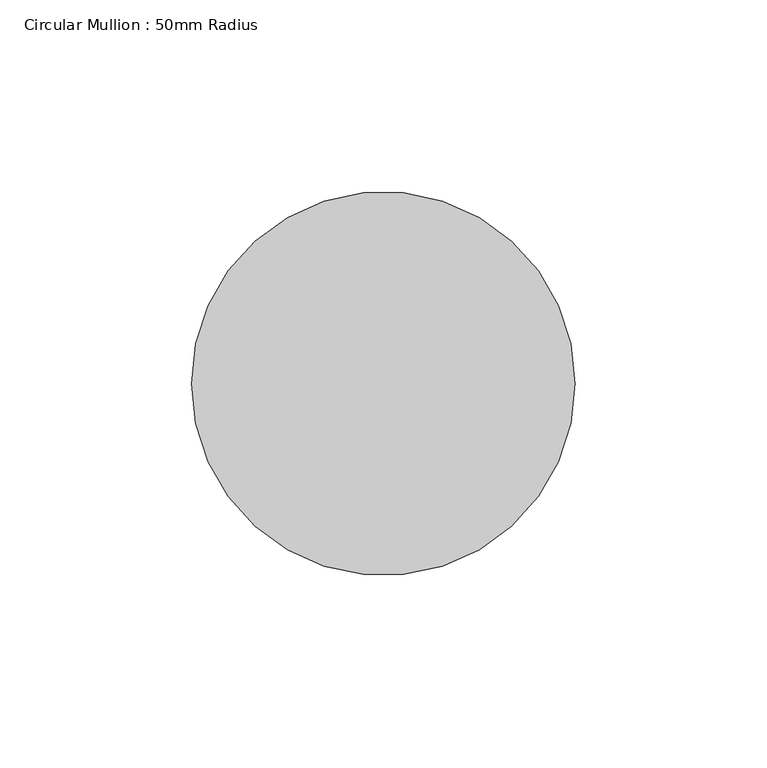
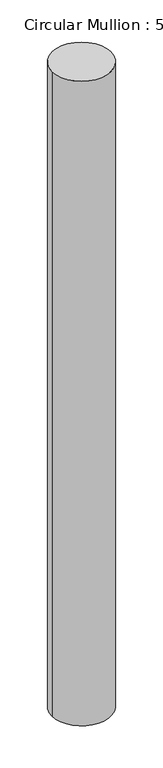
"""IFC4 building model written with IfcOpenShell, lengths in millimetres: member geometry, Circular Mullion : 50mm Radius."""

from ifc_helpers import new_model, si_unit, point, frame, origin, origin_2d, place, context, project, spatial, circle_curve, trimmed, segment, composite_curve, outline, extrude, source, transform, mapped, element, save


def circular_mullion_50mm_radius_acc5950d(model_context):
    return source(origin(), model_context, "Body", "SweptSolid", [
        extrude(outline(composite_curve([segment(trimmed(circle_curve(origin_2d(), 50.0), [point((50.0, 0.0))], [point((-50.0, 0.0))], False, "CARTESIAN"), True, "CONTINUOUS"), segment(trimmed(circle_curve(origin_2d(), 50.0), [point((-50.0, 0.0))], [point((50.0, 0.0))], False, "CARTESIAN"), True, "CONTINUOUS")], self_intersect=False)), frame((0.0, 0.0, -1148.6452152), z_axis=(0.0, 0.0, 1.0), x_axis=(1.0, 0.0, 0.0)), (0.0, 0.0, 1.0), 1148.6452152),
    ])


if __name__ == "__main__":
    model = new_model("IFC4")
    model_context = context("Model", 3, world=origin())
    ifc_project = project(units=[si_unit("LENGTHUNIT", "METRE", prefix="MILLI")], contexts=[model_context])
    site = spatial("IfcSite", under=ifc_project)
    building = spatial("IfcBuilding", under=site)
    placement = place(None, origin())
    circular_mullion_50mm_radius_shape = circular_mullion_50mm_radius_acc5950d(model_context)
    element("IfcMember", 1, ObjectType="Circular Mullion : 50mm Radius", at=placement, inside=building, context=model_context, shape_type="MappedRepresentation", body=[
        mapped(circular_mullion_50mm_radius_shape, transform((0.0, 0.0, 0.0), x_axis=(1.0, 0.0, 0.0), y_axis=(0.0, 1.0, 0.0), z_axis=(0.0, 0.0, 1.0))),
    ])
    save(model, "model.ifc")

# Revit data of these elements
# Type "Circular Mullion : 50mm Radius"
#   built-in parameter 1007350 = 0.164042 (stored number, unit not read)
# Element 1 (IfcMember, "Circular Mullion : 50mm Radius")
#   Materials on its faces: "Aluminium"
# Materials
#   "Aluminium": class "Metal", colour RGB 247 247 247, transparency 0, Description = "Aluminium 6061", Cost = 0
